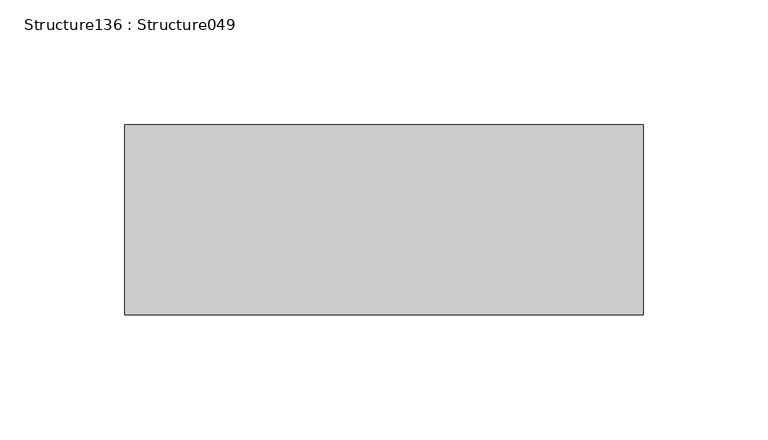
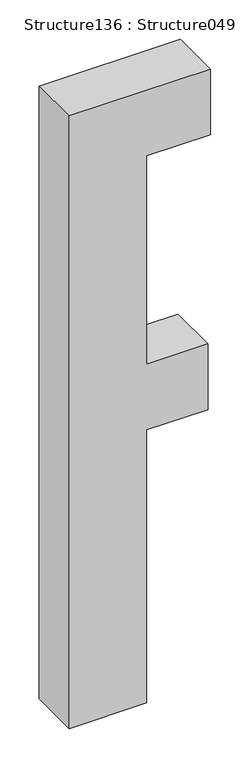
"""IFC4 building model written with IfcOpenShell, lengths in millimetres: proxy geometry, Structure136 : Structure049."""

from ifc_helpers import new_model, si_unit, frame, origin, place, context, project, spatial, polyline, outline, extrude, source, transform, mapped, element, save


def structure136_structure049_4ab7fa26(model_context):
    return source(origin(), model_context, "Body", "SweptSolid", [
        extrude(outline(polyline([(4480.4419946, -48017.328412), (3528.5825142, -48017.328412), (3528.5825142, -47903.0922756), (3952.8367913, -47903.0922756), (3952.8367913, -47813.339045), (4054.8292705, -47813.339045), (4054.8292705, -47903.0922756), (4378.4602217, -47903.0922756), (4378.4602217, -47809.2718911), (4480.4419946, -47809.2718911), (4480.4419946, -48017.328412)])), frame((0.0, 247945.1599557, 0.0), z_axis=(0.0, 1.0, 0.0), x_axis=(0.0, 0.0, 1.0)), (0.0, 0.0, 1.0), 76.2),
    ])


if __name__ == "__main__":
    model = new_model("IFC4")
    model_context = context("Model", 3, world=origin())
    ifc_project = project(units=[si_unit("LENGTHUNIT", "METRE", prefix="MILLI")], contexts=[model_context])
    site = spatial("IfcSite", under=ifc_project)
    building = spatial("IfcBuilding", under=site)
    placement = place(None, origin())
    structure136_structure049_shape = structure136_structure049_4ab7fa26(model_context)
    element("IfcBuildingElementProxy", 1, Name="Structure136 : Structure049", ObjectType="Structure136 : Structure049", at=placement, inside=building, context=model_context, shape_type="MappedRepresentation", body=[
        mapped(structure136_structure049_shape, transform((0.0, 0.0, 0.0), x_axis=(1.0, 0.0, 0.0), y_axis=(0.0, 1.0, 0.0), z_axis=(0.0, 0.0, 1.0))),
    ])
    save(model, "model.ifc")

# Revit data of these elements
# Type "Structure136 : Structure049"
#   NameOverride = "Structure049"
# Element 1 (IfcBuildingElementProxy, "Structure136 : Structure049")
#   Materials on its faces: "BRUSHED ALUM. LETTERING"
# Materials
#   "BRUSHED ALUM. LETTERING": class "Unassigned", colour RGB 169 181 186, transparency 0, Cost = 0
